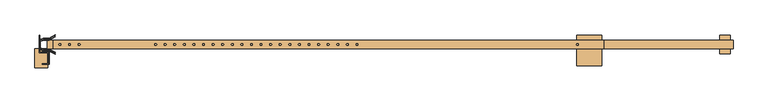
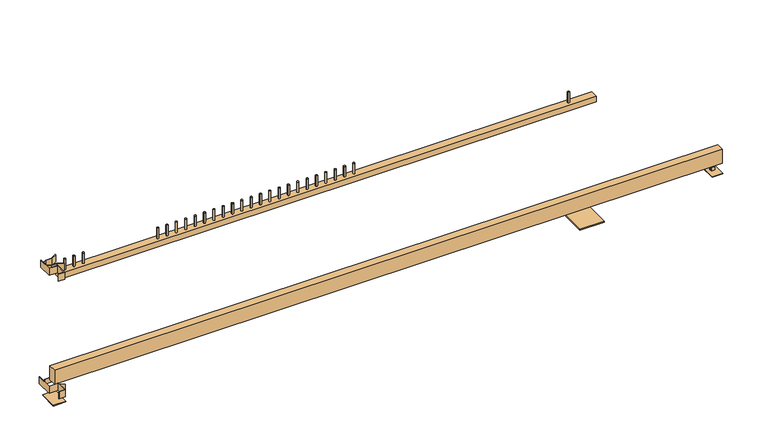
"""IFC4 building model written with IfcOpenShell, lengths in millimetres: door geometry, NLRS_90_DO_UN_schuifpoort met spijlen_gen_rsf : schuifpoort automatisch bxh 7000x1800-NP."""

from ifc_helpers import new_model, si_unit, point, frame, frame_2d, origin, origin_with_axes, place, context, project, spatial, polyline, circle_curve, trimmed, segment, composite_curve, outline, extrude, source, transform, mapped, element, save


def door_02219920(model_context):
    return source(origin(), model_context, "Body", "SweptSolid", [
        extrude(outline(composite_curve([segment(trimmed(circle_curve(frame_2d((-3115.5, 0.0)), 12.5), [point((-3103.0, 0.0))], [point((-3128.0, 0.0))], False, "CARTESIAN"), True, "CONTINUOUS"), segment(trimmed(circle_curve(frame_2d((-3115.5, 0.0)), 12.5), [point((-3128.0, 0.0))], [point((-3103.0, 0.0))], False, "CARTESIAN"), True, "CONTINUOUS")], self_intersect=False)), frame((0.0, 0.0, 1650.0), z_axis=(0.0, 0.0, 1.0), x_axis=(1.0, 0.0, 0.0)), (0.0, 0.0, 1.0), 150.0),
        extrude(outline(composite_curve([segment(trimmed(circle_curve(frame_2d((-3241.5, 0.0)), 12.5), [point((-3229.0, 0.0))], [point((-3254.0, 0.0))], False, "CARTESIAN"), True, "CONTINUOUS"), segment(trimmed(circle_curve(frame_2d((-3241.5, 0.0)), 12.5), [point((-3254.0, 0.0))], [point((-3229.0, 0.0))], False, "CARTESIAN"), True, "CONTINUOUS")], self_intersect=False)), frame((0.0, 0.0, 1650.0), z_axis=(0.0, 0.0, 1.0), x_axis=(1.0, 0.0, 0.0)), (0.0, 0.0, 1.0), 150.0),
        extrude(outline(composite_curve([segment(trimmed(circle_curve(frame_2d((-3367.5, 0.0)), 12.5), [point((-3355.0, 0.0))], [point((-3380.0, 0.0))], False, "CARTESIAN"), True, "CONTINUOUS"), segment(trimmed(circle_curve(frame_2d((-3367.5, 0.0)), 12.5), [point((-3380.0, 0.0))], [point((-3355.0, 0.0))], False, "CARTESIAN"), True, "CONTINUOUS")], self_intersect=False)), frame((0.0, 0.0, 1650.0), z_axis=(0.0, 0.0, 1.0), x_axis=(1.0, 0.0, 0.0)), (0.0, 0.0, 1.0), 150.0),
        extrude(outline(polyline([(3745.0, -280.5), (3415.0, -280.5), (3415.0, 119.5), (3745.0, 119.5), (3745.0, -280.5)])), origin_with_axes(), (0.0, 0.0, 1.0), 12.0),
        extrude(outline(composite_curve([segment(trimmed(circle_curve(frame_2d((3424.5, 0.0)), 12.5), [point((3437.0, 0.0))], [point((3412.0, 0.0))], False, "CARTESIAN"), True, "CONTINUOUS"), segment(trimmed(circle_curve(frame_2d((3424.5, 0.0)), 12.5), [point((3412.0, 0.0))], [point((3437.0, 0.0))], False, "CARTESIAN"), True, "CONTINUOUS")], self_intersect=False)), frame((0.0, 0.0, 1650.0), z_axis=(0.0, 0.0, 1.0), x_axis=(1.0, 0.0, 0.0)), (0.0, 0.0, 1.0), 150.0),
        extrude(outline(composite_curve([segment(trimmed(circle_curve(frame_2d((-727.5, 0.0)), 12.5), [point((-715.0, 0.0))], [point((-740.0, 0.0))], False, "CARTESIAN"), True, "CONTINUOUS"), segment(trimmed(circle_curve(frame_2d((-727.5, 0.0)), 12.5), [point((-740.0, 0.0))], [point((-715.0, 0.0))], False, "CARTESIAN"), True, "CONTINUOUS")], self_intersect=False)), frame((0.0, 0.0, 1650.0), z_axis=(0.0, 0.0, 1.0), x_axis=(1.0, 0.0, 0.0)), (0.0, 0.0, 1.0), 150.0),
        extrude(outline(composite_curve([segment(trimmed(circle_curve(frame_2d((-2111.5, 0.0)), 12.5), [point((-2099.0, 0.0))], [point((-2124.0, 0.0))], False, "CARTESIAN"), True, "CONTINUOUS"), segment(trimmed(circle_curve(frame_2d((-2111.5, 0.0)), 12.5), [point((-2124.0, 0.0))], [point((-2099.0, 0.0))], False, "CARTESIAN"), True, "CONTINUOUS")], self_intersect=False)), frame((0.0, 0.0, 1650.0), z_axis=(0.0, 0.0, 1.0), x_axis=(1.0, 0.0, 0.0)), (0.0, 0.0, 1.0), 150.0),
        extrude(outline(composite_curve([segment(trimmed(circle_curve(frame_2d((531.5, 0.0)), 12.5), [point((544.0, 0.0))], [point((519.0, 0.0))], False, "CARTESIAN"), True, "CONTINUOUS"), segment(trimmed(circle_curve(frame_2d((531.5, 0.0)), 12.5), [point((519.0, 0.0))], [point((544.0, 0.0))], False, "CARTESIAN"), True, "CONTINUOUS")], self_intersect=False)), frame((0.0, 0.0, 1650.0), z_axis=(0.0, 0.0, 1.0), x_axis=(1.0, 0.0, 0.0)), (0.0, 0.0, 1.0), 150.0),
        extrude(outline(composite_curve([segment(trimmed(circle_curve(frame_2d((405.5, 0.0)), 12.5), [point((418.0, 0.0))], [point((393.0, 0.0))], False, "CARTESIAN"), True, "CONTINUOUS"), segment(trimmed(circle_curve(frame_2d((405.5, 0.0)), 12.5), [point((393.0, 0.0))], [point((418.0, 0.0))], False, "CARTESIAN"), True, "CONTINUOUS")], self_intersect=False)), frame((0.0, 0.0, 1650.0), z_axis=(0.0, 0.0, 1.0), x_axis=(1.0, 0.0, 0.0)), (0.0, 0.0, 1.0), 150.0),
        extrude(outline(composite_curve([segment(trimmed(circle_curve(frame_2d((279.5, 0.0)), 12.5), [point((292.0, 0.0))], [point((267.0, 0.0))], False, "CARTESIAN"), True, "CONTINUOUS"), segment(trimmed(circle_curve(frame_2d((279.5, 0.0)), 12.5), [point((267.0, 0.0))], [point((292.0, 0.0))], False, "CARTESIAN"), True, "CONTINUOUS")], self_intersect=False)), frame((0.0, 0.0, 1650.0), z_axis=(0.0, 0.0, 1.0), x_axis=(1.0, 0.0, 0.0)), (0.0, 0.0, 1.0), 150.0),
        extrude(outline(composite_curve([segment(trimmed(circle_curve(frame_2d((153.5, 0.0)), 12.5), [point((166.0, 0.0))], [point((141.0, 0.0))], False, "CARTESIAN"), True, "CONTINUOUS"), segment(trimmed(circle_curve(frame_2d((153.5, 0.0)), 12.5), [point((141.0, 0.0))], [point((166.0, 0.0))], False, "CARTESIAN"), True, "CONTINUOUS")], self_intersect=False)), frame((0.0, 0.0, 1650.0), z_axis=(0.0, 0.0, 1.0), x_axis=(1.0, 0.0, 0.0)), (0.0, 0.0, 1.0), 150.0),
        extrude(outline(composite_curve([segment(trimmed(circle_curve(frame_2d((27.5, 0.0)), 12.5), [point((40.0, 0.0))], [point((15.0, 0.0))], False, "CARTESIAN"), True, "CONTINUOUS"), segment(trimmed(circle_curve(frame_2d((27.5, 0.0)), 12.5), [point((15.0, 0.0))], [point((40.0, 0.0))], False, "CARTESIAN"), True, "CONTINUOUS")], self_intersect=False)), frame((0.0, 0.0, 1650.0), z_axis=(0.0, 0.0, 1.0), x_axis=(1.0, 0.0, 0.0)), (0.0, 0.0, 1.0), 150.0),
        extrude(outline(composite_curve([segment(trimmed(circle_curve(frame_2d((-98.5, 0.0)), 12.5), [point((-86.0, 0.0))], [point((-111.0, 0.0))], False, "CARTESIAN"), True, "CONTINUOUS"), segment(trimmed(circle_curve(frame_2d((-98.5, 0.0)), 12.5), [point((-111.0, 0.0))], [point((-86.0, 0.0))], False, "CARTESIAN"), True, "CONTINUOUS")], self_intersect=False)), frame((0.0, 0.0, 1650.0), z_axis=(0.0, 0.0, 1.0), x_axis=(1.0, 0.0, 0.0)), (0.0, 0.0, 1.0), 150.0),
        extrude(outline(composite_curve([segment(trimmed(circle_curve(frame_2d((-224.5, 0.0)), 12.5), [point((-212.0, 0.0))], [point((-237.0, 0.0))], False, "CARTESIAN"), True, "CONTINUOUS"), segment(trimmed(circle_curve(frame_2d((-224.5, 0.0)), 12.5), [point((-237.0, 0.0))], [point((-212.0, 0.0))], False, "CARTESIAN"), True, "CONTINUOUS")], self_intersect=False)), frame((0.0, 0.0, 1650.0), z_axis=(0.0, 0.0, 1.0), x_axis=(1.0, 0.0, 0.0)), (0.0, 0.0, 1.0), 150.0),
        extrude(outline(composite_curve([segment(trimmed(circle_curve(frame_2d((-350.5, 0.0)), 12.5), [point((-338.0, 0.0))], [point((-363.0, 0.0))], False, "CARTESIAN"), True, "CONTINUOUS"), segment(trimmed(circle_curve(frame_2d((-350.5, 0.0)), 12.5), [point((-363.0, 0.0))], [point((-338.0, 0.0))], False, "CARTESIAN"), True, "CONTINUOUS")], self_intersect=False)), frame((0.0, 0.0, 1650.0), z_axis=(0.0, 0.0, 1.0), x_axis=(1.0, 0.0, 0.0)), (0.0, 0.0, 1.0), 150.0),
        extrude(outline(composite_curve([segment(trimmed(circle_curve(frame_2d((-476.5, 0.0)), 12.5), [point((-464.0, 0.0))], [point((-489.0, 0.0))], False, "CARTESIAN"), True, "CONTINUOUS"), segment(trimmed(circle_curve(frame_2d((-476.5, 0.0)), 12.5), [point((-489.0, 0.0))], [point((-464.0, 0.0))], False, "CARTESIAN"), True, "CONTINUOUS")], self_intersect=False)), frame((0.0, 0.0, 1650.0), z_axis=(0.0, 0.0, 1.0), x_axis=(1.0, 0.0, 0.0)), (0.0, 0.0, 1.0), 150.0),
        extrude(outline(composite_curve([segment(trimmed(circle_curve(frame_2d((-602.5, 0.0)), 12.5), [point((-590.0, 0.0))], [point((-615.0, 0.0))], False, "CARTESIAN"), True, "CONTINUOUS"), segment(trimmed(circle_curve(frame_2d((-602.5, 0.0)), 12.5), [point((-615.0, 0.0))], [point((-590.0, 0.0))], False, "CARTESIAN"), True, "CONTINUOUS")], self_intersect=False)), frame((0.0, 0.0, 1650.0), z_axis=(0.0, 0.0, 1.0), x_axis=(1.0, 0.0, 0.0)), (0.0, 0.0, 1.0), 150.0),
        extrude(outline(composite_curve([segment(trimmed(circle_curve(frame_2d((-852.5, 0.0)), 12.5), [point((-840.0, 0.0))], [point((-865.0, 0.0))], False, "CARTESIAN"), True, "CONTINUOUS"), segment(trimmed(circle_curve(frame_2d((-852.5, 0.0)), 12.5), [point((-865.0, 0.0))], [point((-840.0, 0.0))], False, "CARTESIAN"), True, "CONTINUOUS")], self_intersect=False)), frame((0.0, 0.0, 1650.0), z_axis=(0.0, 0.0, 1.0), x_axis=(1.0, 0.0, 0.0)), (0.0, 0.0, 1.0), 150.0),
        extrude(outline(composite_curve([segment(trimmed(circle_curve(frame_2d((-978.5, 0.0)), 12.5), [point((-966.0, 0.0))], [point((-991.0, 0.0))], False, "CARTESIAN"), True, "CONTINUOUS"), segment(trimmed(circle_curve(frame_2d((-978.5, 0.0)), 12.5), [point((-991.0, 0.0))], [point((-966.0, 0.0))], False, "CARTESIAN"), True, "CONTINUOUS")], self_intersect=False)), frame((0.0, 0.0, 1650.0), z_axis=(0.0, 0.0, 1.0), x_axis=(1.0, 0.0, 0.0)), (0.0, 0.0, 1.0), 150.0),
        extrude(outline(composite_curve([segment(trimmed(circle_curve(frame_2d((-1104.5, 0.0)), 12.5), [point((-1092.0, 0.0))], [point((-1117.0, 0.0))], False, "CARTESIAN"), True, "CONTINUOUS"), segment(trimmed(circle_curve(frame_2d((-1104.5, 0.0)), 12.5), [point((-1117.0, 0.0))], [point((-1092.0, 0.0))], False, "CARTESIAN"), True, "CONTINUOUS")], self_intersect=False)), frame((0.0, 0.0, 1650.0), z_axis=(0.0, 0.0, 1.0), x_axis=(1.0, 0.0, 0.0)), (0.0, 0.0, 1.0), 150.0),
        extrude(outline(composite_curve([segment(trimmed(circle_curve(frame_2d((-1230.5, 0.0)), 12.5), [point((-1218.0, 0.0))], [point((-1243.0, 0.0))], False, "CARTESIAN"), True, "CONTINUOUS"), segment(trimmed(circle_curve(frame_2d((-1230.5, 0.0)), 12.5), [point((-1243.0, 0.0))], [point((-1218.0, 0.0))], False, "CARTESIAN"), True, "CONTINUOUS")], self_intersect=False)), frame((0.0, 0.0, 1650.0), z_axis=(0.0, 0.0, 1.0), x_axis=(1.0, 0.0, 0.0)), (0.0, 0.0, 1.0), 150.0),
        extrude(outline(composite_curve([segment(trimmed(circle_curve(frame_2d((-1356.5, 0.0)), 12.5), [point((-1344.0, 0.0))], [point((-1369.0, 0.0))], False, "CARTESIAN"), True, "CONTINUOUS"), segment(trimmed(circle_curve(frame_2d((-1356.5, 0.0)), 12.5), [point((-1369.0, 0.0))], [point((-1344.0, 0.0))], False, "CARTESIAN"), True, "CONTINUOUS")], self_intersect=False)), frame((0.0, 0.0, 1650.0), z_axis=(0.0, 0.0, 1.0), x_axis=(1.0, 0.0, 0.0)), (0.0, 0.0, 1.0), 150.0),
        extrude(outline(composite_curve([segment(trimmed(circle_curve(frame_2d((-1482.5, 0.0)), 12.5), [point((-1470.0, 0.0))], [point((-1495.0, 0.0))], False, "CARTESIAN"), True, "CONTINUOUS"), segment(trimmed(circle_curve(frame_2d((-1482.5, 0.0)), 12.5), [point((-1495.0, 0.0))], [point((-1470.0, 0.0))], False, "CARTESIAN"), True, "CONTINUOUS")], self_intersect=False)), frame((0.0, 0.0, 1650.0), z_axis=(0.0, 0.0, 1.0), x_axis=(1.0, 0.0, 0.0)), (0.0, 0.0, 1.0), 150.0),
        extrude(outline(composite_curve([segment(trimmed(circle_curve(frame_2d((-1608.5, 0.0)), 12.5), [point((-1596.0, 0.0))], [point((-1621.0, 0.0))], False, "CARTESIAN"), True, "CONTINUOUS"), segment(trimmed(circle_curve(frame_2d((-1608.5, 0.0)), 12.5), [point((-1621.0, 0.0))], [point((-1596.0, 0.0))], False, "CARTESIAN"), True, "CONTINUOUS")], self_intersect=False)), frame((0.0, 0.0, 1650.0), z_axis=(0.0, 0.0, 1.0), x_axis=(1.0, 0.0, 0.0)), (0.0, 0.0, 1.0), 150.0),
        extrude(outline(composite_curve([segment(trimmed(circle_curve(frame_2d((-1734.5, 0.0)), 12.5), [point((-1722.0, 0.0))], [point((-1747.0, 0.0))], False, "CARTESIAN"), True, "CONTINUOUS"), segment(trimmed(circle_curve(frame_2d((-1734.5, 0.0)), 12.5), [point((-1747.0, 0.0))], [point((-1722.0, 0.0))], False, "CARTESIAN"), True, "CONTINUOUS")], self_intersect=False)), frame((0.0, 0.0, 1650.0), z_axis=(0.0, 0.0, 1.0), x_axis=(1.0, 0.0, 0.0)), (0.0, 0.0, 1.0), 150.0),
        extrude(outline(composite_curve([segment(trimmed(circle_curve(frame_2d((-1860.5, 0.0)), 12.5), [point((-1848.0, 0.0))], [point((-1873.0, 0.0))], False, "CARTESIAN"), True, "CONTINUOUS"), segment(trimmed(circle_curve(frame_2d((-1860.5, 0.0)), 12.5), [point((-1873.0, 0.0))], [point((-1848.0, 0.0))], False, "CARTESIAN"), True, "CONTINUOUS")], self_intersect=False)), frame((0.0, 0.0, 1650.0), z_axis=(0.0, 0.0, 1.0), x_axis=(1.0, 0.0, 0.0)), (0.0, 0.0, 1.0), 150.0),
        extrude(outline(composite_curve([segment(trimmed(circle_curve(frame_2d((-1986.5, 0.0)), 12.5), [point((-1974.0, 0.0))], [point((-1999.0, 0.0))], False, "CARTESIAN"), True, "CONTINUOUS"), segment(trimmed(circle_curve(frame_2d((-1986.5, 0.0)), 12.5), [point((-1999.0, 0.0))], [point((-1974.0, 0.0))], False, "CARTESIAN"), True, "CONTINUOUS")], self_intersect=False)), frame((0.0, 0.0, 1650.0), z_axis=(0.0, 0.0, 1.0), x_axis=(1.0, 0.0, 0.0)), (0.0, 0.0, 1.0), 150.0),
        extrude(outline(polyline([(-3430.0, 104.7285156), (-3428.15625, 101.1699219), (-3509.78125, 59.3066406), (-3585.5625, 59.3066406), (-3629.0, 37.0292969), (-3629.0, -37.0332031), (-3585.5625, -59.3105469), (-3509.78125, -59.3105469), (-3428.15625, -101.1738281), (-3430.0, -104.7324219), (-3510.75, -63.3105469), (-3586.53125, -63.3105469), (-3633.0, -39.4707031), (-3633.0, 39.4667969), (-3586.53125, 63.3066406), (-3510.75, 63.3066406), (-3430.0, 104.7285156)])), frame((0.0, 0.0, 1720.0), z_axis=(0.0, 0.0, 1.0), x_axis=(1.0, 0.0, 0.0)), (0.0, 0.0, 1.0), 100.0),
        extrude(outline(polyline([(-3638.0, -105.534128), (-3638.0, 85.4980469), (-3633.0, 85.4980469), (-3633.0, -100.534128), (-3519.015625, -100.534128), (-3519.015625, -260.534128), (-3601.25, -260.534128), (-3601.25, -255.534128), (-3524.015625, -255.534128), (-3524.015625, -105.534128), (-3638.0, -105.534128)])), frame((0.0, 0.0, 1720.0), z_axis=(0.0, 0.0, 1.0), x_axis=(1.0, 0.0, 0.0)), (0.0, 0.0, 1.0), 100.0),
        extrude(outline(composite_curve([segment(polyline([(12.0, 5337.0), (12.0, 5387.0), (42.0, 5387.0)]), True, "CONTINUOUS"), segment(trimmed(circle_curve(frame_2d((42.0, 5362.0)), 25.0), [point((42.0, 5387.0))], [point((42.0, 5337.0))], False, "CARTESIAN"), True, "CONTINUOUS"), segment(polyline([(42.0, 5337.0), (12.0, 5337.0)]), True, "CONTINUOUS")], self_intersect=False)), frame((0.0, -19.0, 0.0), z_axis=(0.0, 1.0, 0.0), x_axis=(0.0, 0.0, 1.0)), (0.0, 0.0, 1.0), 8.0),
        extrude(outline(composite_curve([segment(polyline([(12.0, 5337.0), (12.0, 5387.0), (42.0, 5387.0)]), True, "CONTINUOUS"), segment(trimmed(circle_curve(frame_2d((42.0, 5362.0)), 25.0), [point((42.0, 5387.0))], [point((42.0, 5337.0))], False, "CARTESIAN"), True, "CONTINUOUS"), segment(polyline([(42.0, 5337.0), (12.0, 5337.0)]), True, "CONTINUOUS")], self_intersect=False)), frame((0.0, 11.0, 0.0), z_axis=(0.0, 1.0, 0.0), x_axis=(0.0, 0.0, 1.0)), (0.0, 0.0, 1.0), 8.0),
        extrude(outline(polyline([(5432.0, -120.0), (5292.0, -120.0), (5292.0, 120.0), (5432.0, 120.0), (5432.0, -120.0)])), origin_with_axes(), (0.0, 0.0, 1.0), 12.0),
        extrude(outline(polyline([(5372.0, -11.0), (5352.0, -11.0), (5352.0, 11.0), (5372.0, 11.0), (5372.0, -11.0)])), frame((0.0, 0.0, 12.0), z_axis=(0.0, 0.0, 1.0), x_axis=(1.0, 0.0, 0.0)), (0.0, 0.0, 1.0), 88.0),
        extrude(outline(polyline([(-3429.5, 126.125), (-3427.2114608, 121.6794867), (-3508.5385575, 79.8125), (-3584.542883, 79.8125), (-3628.0, 57.5306685), (-3628.0, -57.5306685), (-3584.542883, -79.8125), (-3508.5385575, -79.8125), (-3427.2114608, -121.6794867), (-3429.5, -126.125), (-3509.75, -84.8125), (-3585.75, -84.8125), (-3633.0, -60.585938), (-3633.0, 60.585938), (-3585.75, 84.8125), (-3509.75, 84.8125), (-3429.5, 126.125)])), frame((0.0, 0.0, 39.0), z_axis=(0.0, 0.0, 1.0), x_axis=(1.0, 0.0, 0.0)), (0.0, 0.0, 1.0), 70.0),
        extrude(outline(polyline([(-3638.0, -105.5), (-3638.0, 119.5), (-3633.0, 119.5), (-3633.0, -100.5), (-3510.0, -100.5), (-3510.0, -260.5), (-3593.0, -260.5), (-3593.0, -255.5), (-3515.0, -255.5), (-3515.0, -105.5), (-3638.0, -105.5)])), frame((0.0, 0.0, 39.0), z_axis=(0.0, 0.0, 1.0), x_axis=(1.0, 0.0, 0.0)), (0.0, 0.0, 1.0), 100.0),
        extrude(outline(polyline([(5467.0, -55.0), (-3535.5, -55.0), (-3535.5, 55.0), (5467.0, 55.0), (5467.0, -55.0)])), frame((0.0, 0.0, 100.0), z_axis=(0.0, 0.0, 1.0), x_axis=(1.0, 0.0, 0.0)), (0.0, 0.0, 1.0), 200.0),
        extrude(outline(polyline([(-3525.0, -305.0), (-3695.0, -305.0), (-3695.0, -55.0), (-3525.0, -55.0), (-3525.0, -305.0)])), origin_with_axes(), (0.0, 0.0, 1.0), 12.0),
        extrude(outline(polyline([(3767.5, -55.0), (-3455.5, -55.0), (-3455.5, 55.0), (3767.5, 55.0), (3767.5, -55.0)])), frame((0.0, 0.0, 1570.0), z_axis=(0.0, 0.0, 1.0), x_axis=(1.0, 0.0, 0.0)), (0.0, 0.0, 1.0), 80.0),
    ])


if __name__ == "__main__":
    model = new_model("IFC4")
    model_context = context("Model", 3, world=origin())
    ifc_project = project(units=[si_unit("LENGTHUNIT", "METRE", prefix="MILLI")], contexts=[model_context])
    site = spatial("IfcSite", under=ifc_project)
    building = spatial("IfcBuilding", under=site)
    placement = place(None, origin())
    door_shape = door_02219920(model_context)
    element("IfcDoor", 1, ObjectType="NLRS_90_DO_UN_schuifpoort met spijlen_gen_rsf : schuifpoort automatisch bxh 7000x1800-NP", at=placement, inside=building, context=model_context, shape_type="MappedRepresentation", body=[
        mapped(door_shape, transform((0.0, 0.0, 0.0), x_axis=(1.0, 0.0, 0.0), y_axis=(0.0, 1.0, 0.0), z_axis=(0.0, 0.0, 1.0))),
    ])
    save(model, "model.ifc")

# Revit data of these elements
# Project information
#   Organization Name = "RSF"
#   Organization Description = "Revit Standards Foundation"
#   Building Name = "Onderwijsmodel Bouwkundig"
#   Author = "Emiel Ham TC-lid NLRS"
#   NLRS_C_opdrachtgever_adres = "Het Zuiderkruis 17, 5215 MV, 's-Hertogenbosch"
#   NLRS_C_opdrachtgever_contactpersoon = "Bestuur RSF"
#   NLRS_C_opdrachtgever_email = "secretary@revitstandards.org"
#   NLRS_C_opdrachtgever_projectnummer = "2017.4.015"
#   NLRS_C_opdrachtgever_telefoon = "nvt"
#   NLRS_C_project_email = "tc@revitstandards.org"
#   NLRS_C_project_kadaster_gemeente = "BIMSTAD"
#   NLRS_C_project_kadaster_nummer = "3"
#   NLRS_C_project_kadaster_sectie = "D"
#   NLRS_C_project_projectleider = "Martijn de Riet"
#   NLRS_C_project_telefoon = "+316 24 28 31 75"
#   NLRS_C_leverancier_bedrijfsnaam = "Technische Commissie RSF"
#   NLRS_C_leverancier_adres = "Het Zuiderkruis 17"
#   NLRS_C_leverancier_postcode = "5215 MV"
#   NLRS_C_leverancier_plaats = "'s-Hertogenbosch"
#   NLRS_C_leverancier_telefoonnummer = "nvt"
#   NLRS_C_leverancier_fax = "nvt"
#   NLRS_C_leverancier_email = "tc@revitstandards.org"
#   Workset = "Project Info"
#   IfcSite GUID = "3a0_Qb3mb9RuT4Z3SQBcsf"
#   IfcBuilding GUID = "3a0_Qb3mb9RuT4Z3SQBcsg"
#   IfcProject GUID = "3a0_Qb3mb9RuT4Z3SQBcsh"
#   Project Issue Date = "07-10-2021"
#   Project Status = "DEFINITIEF"
#   Client Name = "Revit Standards Foundation"
#   Project Address = "Onderwijsboulevard 123\n4567 HI Bimstad"
#   Project Name = "Onderwijsmodellen NLRS"
#   Project Number = "Onderwijsmodellen"
#   BCB_ProjectFolder = "C:\\Users\\Martijn de Riet\\Documents\\2023"
# Type "NLRS_90_DO_UN_schuifpoort met spijlen_gen_rsf : schuifpoort automatisch bxh 7000x1800-NP"
#   Type IFC Predefined Type = "GATE"
#   Export Type to IFC As = "IfcDoorType"
#   Type IfcGUID = "1A81voHkv98RYujw6ZYnX6"
#   IfcName[Type] = "schuifpoort automatisch bxh 7000x1800-NP"
#   IfcDescription[Type] = "schuifpoort doorgang bxh 7000x1800mm"
#   IfcExportAs[Type] = "IfcDoorType"
#   IfcExportType[Type] = "GATE"
#   NLRS_C_revit_versie = ""
#   NLRS_C_omschrijving_03 [instance default] = "doorgangsmaat"
#   NLRS_C_omschrijving_02 [instance default] = "stootplaat"
#   NLRS_C_omschrijving_01 [instance default] = "rolpoort"
#   NLRS_C_content_versie = ""
#   NLRS_C_content_provider = ""
#   NLRS_C_content_handleiding = ""
#   NLRS_C_content_datum_uitgifte = ""
#   NLRS_C_content_datum_gewijzigd = ""
#   NLRS_C_content_creator = ""
#   Model = "generiek"
#   Manufacturer = "Revit Standards Foundation"
#   Description = "schuifpoort doorgang bxh 7000x1800mm"
#   Assembly Code = "90.32"
#   NLRS_C_hoogte = 1800.00 mm
#   NLRS_C_breedte_03 = 7000.00 mm
#   NLRS_C_materiaal_02 = NLRS_n5_rubber_gen_bf
#   NLRS_C_materiaal_01 = NLRS_h4_aluminium 250-255-255_gen_rsf
#   URL = ""
#   Keynote = ""
#   Default Elevation = 0
# Element 1 (IfcDoor, "NLRS_90_DO_UN_schuifpoort met spijlen_gen_rsf : schuifpoort automatisch bxh 7000x1800-NP")
#   Materials on its faces: "NLRS_h4_aluminium 250-255-255_gen_rsf", "NLRS_n5_rubber_gen_bf"
# Materials
#   "NLRS_n5_rubber_gen_bf": class "N - Kunststoffen, rubbers", colour RGB 63 63 63, transparency 0, Keynote = "n5", Model = "generiek", Manufacturer = "Revit Standards Foundation", URL = "www.revitstandards.org", Description = "rubber daktegels 600x600mm", Cost = 0
#   "NLRS_h4_aluminium 250-255-255_gen_rsf": class "BCB class", colour RGB 250 255 255, transparency 0, Keynote = "h4", Model = "generiek", Manufacturer = "Revit Standards Foundation", URL = "www.revitstandards.org", Description = "aluminium wit", Cost = 0
